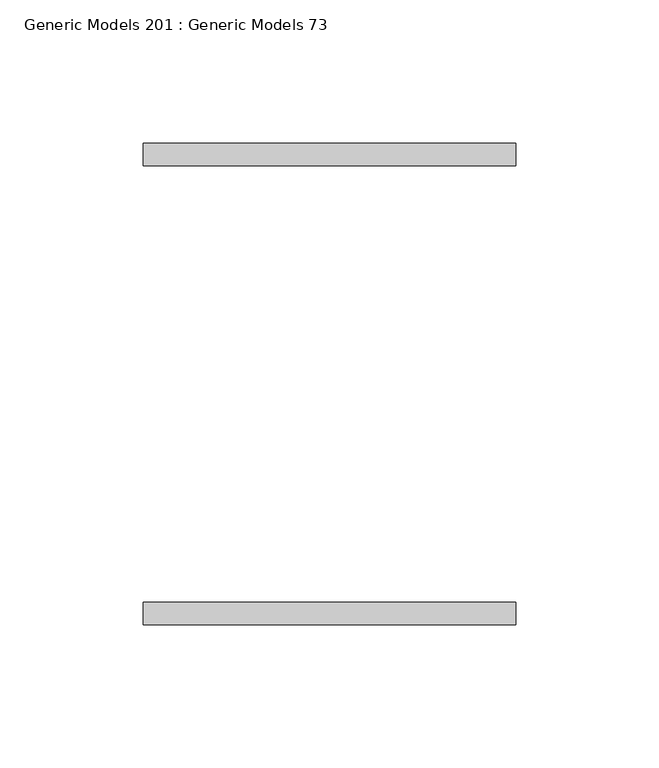
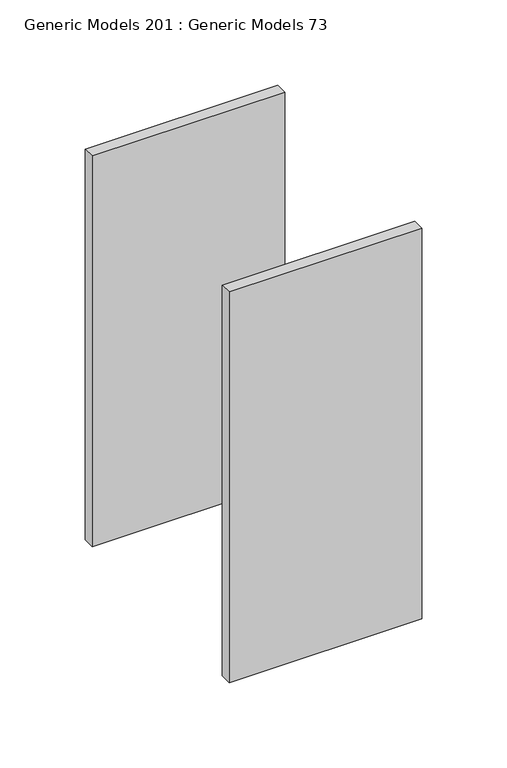
"""IFC4 building model written with IfcOpenShell, lengths in millimetres: proxy geometry, Generic Models 201 : Generic Models 73."""

from ifc_helpers import new_model, si_unit, frame, origin, place, context, project, spatial, polyline, outline, extrude, source, transform, mapped, element, save


def generic_models_201_generic_models_73_2826c1c3(model_context):
    return source(origin(), model_context, "Body", "SweptSolid", [
        extrude(outline(polyline([(32040.4971032, 36491.5582942), (32040.4971032, 36483.6207942), (31910.3221032, 36483.6207942), (31910.3221032, 36491.5582942), (32040.4971032, 36491.5582942)])), frame((0.0, 0.0, 269146.3375), z_axis=(0.0, 0.0, 1.0), x_axis=(1.0, 0.0, 0.0)), (0.0, 0.0, 1.0), 279.4),
        extrude(outline(polyline([(32040.4971032, 36331.2207942), (32040.4971032, 36323.2832942), (31910.3221032, 36323.2832942), (31910.3221032, 36331.2207942), (32040.4971032, 36331.2207942)])), frame((0.0, 0.0, 269146.3375), z_axis=(0.0, 0.0, 1.0), x_axis=(1.0, 0.0, 0.0)), (0.0, 0.0, 1.0), 279.4),
    ])


if __name__ == "__main__":
    model = new_model("IFC4")
    model_context = context("Model", 3, world=origin())
    ifc_project = project(units=[si_unit("LENGTHUNIT", "METRE", prefix="MILLI")], contexts=[model_context])
    site = spatial("IfcSite", under=ifc_project)
    building = spatial("IfcBuilding", under=site)
    placement = place(None, origin())
    generic_models_201_generic_models_73_shape = generic_models_201_generic_models_73_2826c1c3(model_context)
    element("IfcBuildingElementProxy", 1, Name="Generic Models 201 : Generic Models 73", ObjectType="Generic Models 201 : Generic Models 73", at=placement, inside=building, context=model_context, shape_type="MappedRepresentation", body=[
        mapped(generic_models_201_generic_models_73_shape, transform((0.0, 0.0, 0.0), x_axis=(1.0, 0.0, 0.0), y_axis=(0.0, 1.0, 0.0), z_axis=(0.0, 0.0, 1.0))),
    ])
    save(model, "model.ifc")

# Revit data of these elements
# Element 1 (IfcBuildingElementProxy, "Generic Models 201 : Generic Models 73")
#   Materials on its faces: "5/16 x 9 x 0'-11\" SIDE PLATES  CAP\nW/ 2 3/4\"DIA. THRU BOLTS"
# Materials
#   "5/16 x 9 x 0'-11\" SIDE PLATES  CAP\nW/ 2 3/4\"DIA. THRU BOLTS": class "Metal", colour RGB 199 199 199, transparency 0, Description = "Carbon steel", Cost = 0
